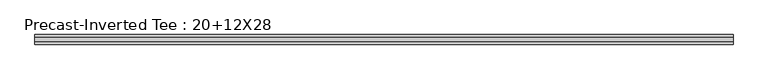
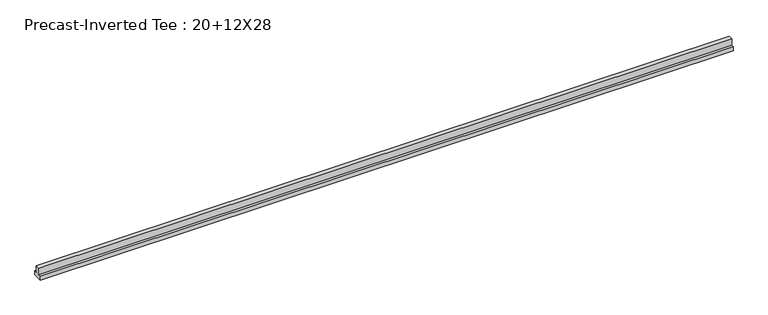
"""IFC4 building model written with IfcOpenShell, lengths in millimetres: beam geometry, Precast-Inverted Tee : 20+12X28."""

from ifc_helpers import new_model, si_unit, frame, origin, place, context, project, spatial, polyline, outline, extrude, source, transform, mapped, element, save


def precast_inverted_tee_20_12x28_ea35af0b(model_context):
    return source(origin(), model_context, "Body", "SweptSolid", [
        extrude(outline(polyline([(-355.6, -406.4), (-355.6, -101.6), (-152.4, -101.6), (-152.4, 406.4), (152.4, 406.4), (152.4, -101.6), (355.6, -101.6), (355.6, -406.4), (-355.6, -406.4)])), frame((-25831.8, 0.0, 0.0), z_axis=(1.0, 0.0, 0.0), x_axis=(0.0, 1.0, 0.0)), (0.0, 0.0, 1.0), 51587.4),
    ])


if __name__ == "__main__":
    model = new_model("IFC4")
    model_context = context("Model", 3, world=origin())
    ifc_project = project(units=[si_unit("LENGTHUNIT", "METRE", prefix="MILLI")], contexts=[model_context])
    site = spatial("IfcSite", under=ifc_project)
    building = spatial("IfcBuilding", under=site)
    placement = place(None, origin())
    precast_inverted_tee_20_12x28_shape = precast_inverted_tee_20_12x28_ea35af0b(model_context)
    element("IfcBeam", 1, ObjectType="Precast-Inverted Tee : 20+12X28", at=placement, inside=building, context=model_context, shape_type="MappedRepresentation", body=[
        mapped(precast_inverted_tee_20_12x28_shape, transform((0.0, 0.0, 0.0), x_axis=(1.0, 0.0, 0.0), y_axis=(0.0, 1.0, 0.0), z_axis=(0.0, 0.0, 1.0))),
    ])
    save(model, "model.ifc")

# Revit data of these elements
# Type "Precast-Inverted Tee : 20+12X28"
#   Assembly Code = "B10"
#   Seat = 0' - 8"
#   Length [instance default] = 5' - 0"
#   b = 2' - 4"
#   h = 2' - 8"
#   h1 = 1' - 8"
#   Structural Material [instance default] = Concrete - Precast Concrete - Normal Weight Concrete - 5 ksi
# Element 1 (IfcBeam, "Precast-Inverted Tee : 20+12X28")
#   Length = 169' - 6"
#   Materials on its faces: "Concrete - Precast Concrete - Normal Weight Concrete - 5 ksi"
# Materials
#   "Concrete - Precast Concrete - Normal Weight Concrete - 5 ksi": class "Concrete", colour RGB 198 187 187, transparency 0, Cost = 0
